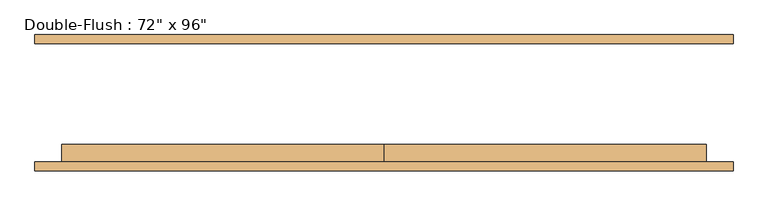
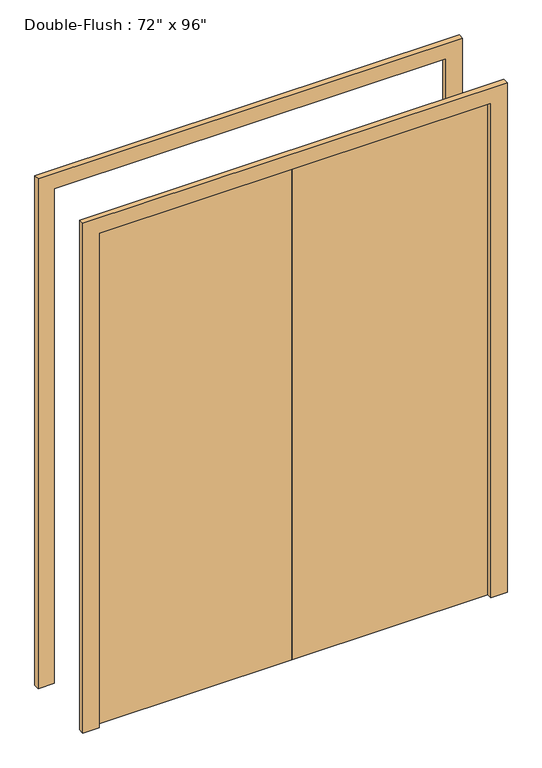
"""IFC4 building model written with IfcOpenShell, lengths in millimetres: door geometry."""

from ifc_helpers import new_model, si_unit, frame, origin, origin_with_axes, place, context, project, spatial, polyline, outline, extrude, source, transform, mapped, element, save


def door_92b4c88e(model_context):
    return source(origin(), model_context, "Body", "SweptSolid", [
        extrude(outline(polyline([(0.0, -168.275), (0.0, -117.475), (914.4, -117.475), (914.4, -168.275), (0.0, -168.275)])), origin_with_axes(), (0.0, 0.0, 1.0), 2438.4),
        extrude(outline(polyline([(-914.4, -168.275), (-914.4, -117.475), (0.0, -117.475), (0.0, -168.275), (-914.4, -168.275)])), origin_with_axes(), (0.0, 0.0, 1.0), 2438.4),
        extrude(outline(polyline([(2438.4, -914.4), (2438.4, 914.4), (0.0, 914.4), (0.0, 990.6), (2514.6, 990.6), (2514.6, -990.6), (0.0, -990.6), (0.0, -914.4), (2438.4, -914.4)])), frame((0.0, 168.275, 0.0), z_axis=(0.0, 1.0, 0.0), x_axis=(0.0, 0.0, 1.0)), (0.0, 0.0, 1.0), 25.4),
        extrude(outline(polyline([(2438.4, -914.4), (2438.4, 914.4), (0.0, 914.4), (0.0, 990.6), (2514.6, 990.6), (2514.6, -990.6), (0.0, -990.6), (0.0, -914.4), (2438.4, -914.4)])), frame((0.0, -193.675, 0.0), z_axis=(0.0, 1.0, 0.0), x_axis=(0.0, 0.0, 1.0)), (0.0, 0.0, 1.0), 25.4),
    ])


if __name__ == "__main__":
    model = new_model("IFC4")
    model_context = context("Model", 3, world=origin())
    ifc_project = project(units=[si_unit("LENGTHUNIT", "METRE", prefix="MILLI")], contexts=[model_context])
    site = spatial("IfcSite", under=ifc_project)
    building = spatial("IfcBuilding", under=site)
    placement = place(None, origin())
    door_shape = door_92b4c88e(model_context)
    element("IfcDoor", 1, ObjectType="Double-Flush : 72\" x 96\"", at=placement, inside=building, context=model_context, shape_type="MappedRepresentation", body=[
        mapped(door_shape, transform((0.0, 0.0, 0.0), x_axis=(1.0, 0.0, 0.0), y_axis=(0.0, 1.0, 0.0), z_axis=(0.0, 0.0, 1.0))),
    ])
    save(model, "model.ifc")

# Revit data of these elements
# Type "Double-Flush : 72\" x 96\""
#   Type Mark = "38"
#   Construction Type Id = "MDOOR"
#   Assembly Code = "C1020"
#   Analytic Construction = "Metal"
#   Thickness = 0' - 2"
#   Heat Transfer Coefficient (U) = 3.7021 W/(m²·K)
#   Height = 8' - 0"
#   Trim Projection Ext = 0' - 1"
#   Trim Projection Int = 0' - 1"
#   Trim Width = 0' - 3"
#   Width = 6' - 0"
#   Door Material = INTERIOR GRADE ALUMINUM STOREFRONT W/ SAFETY GLAZING
#   Frame Material = INTERIOR GRADE ALUMINUM STOREFRONT W/ SAFETY GLAZING
#   Visual Light Transmittance = 0
#   Solar Heat Gain Coefficient = 0
#   Function = (empty or 0)
#   Wall Closure = (empty or 0)
# Element 1 (IfcDoor, "Double-Flush : 72\" x 96\"")
#   Materials on its faces: "INTERIOR GRADE ALUMINUM STOREFRONT W/ SAFETY GLAZING"
# Materials
#   "INTERIOR GRADE ALUMINUM STOREFRONT W/ SAFETY GLAZING": class "Metal", colour RGB 226 226 226, transparency 0, Description = "Aluminum 6061", Cost = 0
